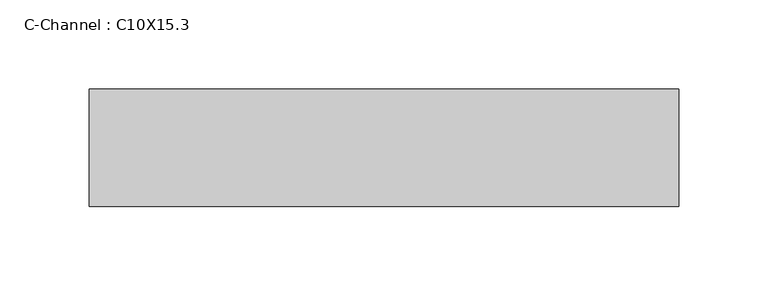
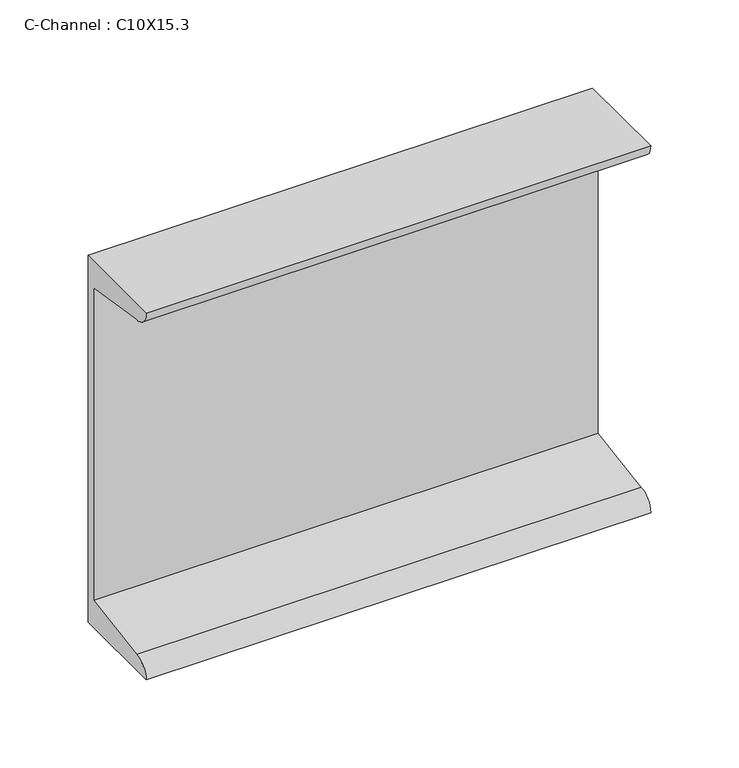
"""IFC4 building model written with IfcOpenShell, lengths in millimetres: beam geometry, C-Channel : C10X15.3."""

import ifcopenshell
import ifcopenshell.guid

model = None  # the IFC model being written
_history = None  # IfcOwnerHistory: only IFC2X3 demands one
_inside = {}  # id of a spatial element -> (the spatial element, [elements in it])
_under = {}  # id of a project, library or spatial element -> (it, [spatial elements below it])
_declared = {}  # id of a project -> (the project, [libraries it declares])
_typed = {}  # id of a type object -> (the type object, [elements of that type])
_made_of = {}  # id of a material, layer set ... -> (it, [elements and type objects made of it])


def new_model(schema):
    """Start an empty IFC model of exactly this schema.

    Asked for "IFC4X3", IfcOpenShell would pick the latest addendum, in which some entities
    have other attributes; the version numbers below select the first issue.
    IFC2X3 requires an IfcOwnerHistory on every rooted entity: one is made here for all.
    """
    global model, _history
    if schema == "IFC4X3":
        model = ifcopenshell.file(schema_version=(4, 3, 0, 0))
    else:
        model = ifcopenshell.file(schema=schema)
    _inside.clear()
    _under.clear()
    _declared.clear()
    _typed.clear()
    _made_of.clear()
    _history = None
    if model.schema == "IFC2X3":
        org = make("IfcOrganization", Name="unknown")
        user = make(
            "IfcPersonAndOrganization",
            ThePerson=make("IfcPerson", FamilyName="unknown"),
            TheOrganization=org,
        )
        app = make(
            "IfcApplication",
            ApplicationDeveloper=org,
            Version="unknown",
            ApplicationFullName="unknown",
            ApplicationIdentifier="unknown",
        )
        _history = make(
            "IfcOwnerHistory",
            OwningUser=user,
            OwningApplication=app,
            ChangeAction="ADDED",
            CreationDate=0,
        )
    return model


def make(cls, **values):
    """One entity of the class cls with the attributes given. An attribute that is None is left unset."""
    return model.create_entity(
        cls, **{name: value for name, value in values.items() if value is not None}
    )


def rooted(cls, **values):
    """An entity with a GlobalId (a new one), such as an element, a storey or a relation."""
    return make(cls, GlobalId=ifcopenshell.guid.new(), OwnerHistory=_history, **values)


def si_unit(unit_type, name, prefix=None):
    """IfcSIUnit, for example si_unit("LENGTHUNIT", "METRE", prefix="MILLI")."""
    return make("IfcSIUnit", UnitType=unit_type, Prefix=prefix, Name=name)


def assignment(units):
    """IfcUnitAssignment: the units of a project."""
    return None if units is None else make("IfcUnitAssignment", Units=units)


def point(xyz):
    """IfcCartesianPoint."""
    return None if xyz is None else make("IfcCartesianPoint", Coordinates=xyz)


def direction(xyz):
    """IfcDirection."""
    return None if xyz is None else make("IfcDirection", DirectionRatios=xyz)


def frame(location, z_axis=None, x_axis=None):
    """IfcAxis2Placement3D, a coordinate frame: its origin and axes. An axis left out is left unset."""
    return make(
        "IfcAxis2Placement3D",
        Location=point(location),
        Axis=direction(z_axis),
        RefDirection=direction(x_axis),
    )


def frame_2d(location, x_axis=None):
    """IfcAxis2Placement2D, a coordinate frame in the plane: its origin and x axis."""
    return make(
        "IfcAxis2Placement2D", Location=point(location), RefDirection=direction(x_axis)
    )


def origin():
    """The frame at (0, 0, 0) with its axes left unset."""
    return frame((0.0, 0.0, 0.0))


def place(relative_to, where):
    """IfcLocalPlacement: puts the frame where relative to a parent placement (None: the world)."""
    return make(
        "IfcLocalPlacement", PlacementRelTo=relative_to, RelativePlacement=where
    )


def context(
    kind, dimensions, precision=None, world=None, true_north=None, identifier=None
):
    """IfcGeometricRepresentationContext, for example the 3D "Model" context."""
    return make(
        "IfcGeometricRepresentationContext",
        ContextIdentifier=identifier,
        ContextType=kind,
        CoordinateSpaceDimension=dimensions,
        Precision=precision,
        WorldCoordinateSystem=world,
        TrueNorth=true_north,
    )


def project(units=None, contexts=None):
    """IfcProject with its units and contexts."""
    return rooted(
        "IfcProject",
        Name="project",
        RepresentationContexts=contexts,
        UnitsInContext=assignment(units),
    )


def spatial(cls, under=None, at=None, **own):
    """A site, building, storey or space (cls), placed at a placement, below another one or the project."""
    s = rooted(cls, ObjectPlacement=at, **own)
    if under is not None:
        _under.setdefault(under.id(), (under, []))[1].append(s)
    return s


def polyline(points):
    """IfcPolyline through the points."""
    return make("IfcPolyline", Points=[point(p) for p in points])


def circle_curve(where, radius):
    """IfcCircle in the frame where."""
    return make("IfcCircle", Position=where, Radius=radius)


def trimmed(basis, trim1, trim2, sense, master):
    """IfcTrimmedCurve: the piece of a basis curve between two trims."""
    return make(
        "IfcTrimmedCurve",
        BasisCurve=basis,
        Trim1=trim1,
        Trim2=trim2,
        SenseAgreement=sense,
        MasterRepresentation=master,
    )


def segment(curve, same_sense, transition):
    """IfcCompositeCurveSegment."""
    return make(
        "IfcCompositeCurveSegment",
        Transition=transition,
        SameSense=same_sense,
        ParentCurve=curve,
    )


def composite_curve(segments, self_intersect=None):
    """IfcCompositeCurve: segments joined end to end."""
    return make("IfcCompositeCurve", Segments=segments, SelfIntersect=self_intersect)


def outline(outer, holes=None, kind="AREA"):
    """IfcArbitraryClosedProfileDef: a profile drawn as a closed curve; with holes, ...WithVoids."""
    if holes is None:
        return make("IfcArbitraryClosedProfileDef", ProfileType=kind, OuterCurve=outer)
    return make(
        "IfcArbitraryProfileDefWithVoids",
        ProfileType=kind,
        OuterCurve=outer,
        InnerCurves=holes,
    )


def extrude(swept, where, along, depth):
    """IfcExtrudedAreaSolid: the profile swept, set in the frame where, extruded along a direction by depth."""
    return make(
        "IfcExtrudedAreaSolid",
        SweptArea=swept,
        Position=where,
        ExtrudedDirection=direction(along),
        Depth=depth,
    )


def shape(context_of_items, identifier, shape_type, items):
    """IfcShapeRepresentation: the items that make up one representation, for example the "Body"."""
    return make(
        "IfcShapeRepresentation",
        ContextOfItems=context_of_items,
        RepresentationIdentifier=identifier,
        RepresentationType=shape_type,
        Items=items,
    )


def source(mapping_origin, context_of_items, identifier, shape_type, items):
    """IfcRepresentationMap: a shape defined once, which mapped items show again and again."""
    return make(
        "IfcRepresentationMap",
        MappingOrigin=mapping_origin,
        MappedRepresentation=shape(context_of_items, identifier, shape_type, items),
    )


def transform(
    local_origin,
    x_axis=None,
    y_axis=None,
    z_axis=None,
    scale=None,
    scale2=None,
    scale3=None,
    uniform=True,
):
    """IfcCartesianTransformationOperator3D, or its non-uniform kind. x_axis, y_axis, z_axis: its Axis1, 2, 3."""
    if uniform:
        return make(
            "IfcCartesianTransformationOperator3D",
            Axis1=direction(x_axis),
            Axis2=direction(y_axis),
            LocalOrigin=point(local_origin),
            Scale=scale,
            Axis3=direction(z_axis),
        )
    return make(
        "IfcCartesianTransformationOperator3DnonUniform",
        Axis1=direction(x_axis),
        Axis2=direction(y_axis),
        LocalOrigin=point(local_origin),
        Scale=scale,
        Axis3=direction(z_axis),
        Scale2=scale2,
        Scale3=scale3,
    )


def mapped(mapping_source, mapping_target):
    """IfcMappedItem: shows the shape of a source again, moved by a transform."""
    return make(
        "IfcMappedItem", MappingSource=mapping_source, MappingTarget=mapping_target
    )


def made_of(thing, what):
    """Note that an element or type object is made of a material, layer set ...; save() writes the relation."""
    if what is not None:
        _made_of.setdefault(what.id(), (what, []))[1].append(thing)
    return thing


def element(
    cls,
    number,
    at=None,
    inside=None,
    cuts=None,
    type_object=None,
    material=None,
    context=None,
    identifier="Body",
    shape_type=None,
    held_by="IfcProductDefinitionShape",
    body=None,
    shapes=None,
    **own,
):
    """One element of the class cls, such as IfcWall. Its Tag is "e" and its number.

    at: its placement. inside: the storey or other place that contains it. cuts: it is an
    opening in that element (IfcRelVoidsElement). A single representation is given by context,
    identifier, shape_type and body (its items); several are given by shapes. held_by: the class
    of the entity that holds the representations. save() writes the other relations.
    """
    e = rooted(cls, Tag="e%d" % number, ObjectPlacement=at, **own)
    if body is not None:
        shapes = [shape(context, identifier, shape_type, body)]
    if shapes is not None:
        e.Representation = make(held_by, Representations=shapes)
    if inside is not None:
        _inside.setdefault(inside.id(), (inside, []))[1].append(e)
    if cuts is not None:
        rooted(
            "IfcRelVoidsElement", RelatingBuildingElement=cuts, RelatedOpeningElement=e
        )
    if type_object is not None:
        _typed.setdefault(type_object.id(), (type_object, []))[1].append(e)
    return made_of(e, material)


def aggregate(whole, parts):
    """IfcRelAggregates: a whole, such as a stair, and the parts it consists of."""
    return rooted("IfcRelAggregates", RelatingObject=whole, RelatedObjects=parts)


def save(model, path):
    """Write the relations noted so far, then the file.

    IfcRelAggregates (storeys below a building ...), IfcRelContainedInSpatialStructure (elements
    in a storey), IfcRelDefinesByType, IfcRelAssociatesMaterial and IfcRelDeclares: one each for
    every whole, place, type object, material and project.
    """
    for whole, parts in _under.values():
        aggregate(whole, parts)
    for where, things in _inside.values():
        rooted(
            "IfcRelContainedInSpatialStructure",
            RelatedElements=things,
            RelatingStructure=where,
        )
    for kind, things in _typed.values():
        rooted("IfcRelDefinesByType", RelatedObjects=things, RelatingType=kind)
    for what, things in _made_of.values():
        rooted("IfcRelAssociatesMaterial", RelatedObjects=things, RelatingMaterial=what)
    for by, libraries in _declared.values():
        rooted("IfcRelDeclares", RelatingContext=by, RelatedDefinitions=libraries)
    model.write(path)


def c_channel_c10x15_3_927e855d(model_context):
    return source(origin(), model_context, "Body", "SweptSolid", [
        extrude(outline(composite_curve([segment(polyline([(16.1036, 127.0), (16.1036, -127.0), (-49.9364, -127.0)]), True, "CONTINUOUS"), segment(trimmed(circle_curve(frame_2d((-38.862, -127.0)), 11.0744), [point((-49.9364, -127.0))], [point((-38.862, -115.9256))], False, "CARTESIAN"), True, "CONTINUOUS"), segment(polyline([(-38.862, -115.9256), (10.0076, -108.1854158), (10.0076, 108.1854158), (-38.862, 115.9256)]), True, "CONTINUOUS"), segment(trimmed(circle_curve(frame_2d((-38.862, 127.0)), 11.0744), [point((-38.862, 115.9256))], [point((-49.9364, 127.0))], False, "CARTESIAN"), True, "CONTINUOUS"), segment(polyline([(-49.9364, 127.0), (16.1036, 127.0)]), True, "CONTINUOUS")], self_intersect=False)), frame((-178.308, 0.0, 0.0), z_axis=(1.0, 0.0, 0.0), x_axis=(0.0, 1.0, 0.0)), (0.0, 0.0, 1.0), 330.708),
    ])


if __name__ == "__main__":
    model = new_model("IFC4")
    model_context = context("Model", 3, world=origin())
    ifc_project = project(units=[si_unit("LENGTHUNIT", "METRE", prefix="MILLI")], contexts=[model_context])
    site = spatial("IfcSite", under=ifc_project)
    building = spatial("IfcBuilding", under=site)
    placement = place(None, origin())
    c_channel_c10x15_3_shape = c_channel_c10x15_3_927e855d(model_context)
    element("IfcBeam", 1, ObjectType="C-Channel : C10X15.3", at=placement, inside=building, context=model_context, shape_type="MappedRepresentation", body=[
        mapped(c_channel_c10x15_3_shape, transform((0.0, 0.0, 0.0), x_axis=(1.0, 0.0, 0.0), y_axis=(0.0, 1.0, 0.0), z_axis=(0.0, 0.0, 1.0))),
    ])
    save(model, "model.ifc")

# Revit data of these elements
# Type "C-Channel : C10X15.3"
#   Assembly Code = "B10"
#   W = 15.3
#   Length [instance default] = 5' - 0"
#   bf = 0' - 2.6"
#   d = 0' - 10"
#   tf = 0' - 0.436"
#   tw = 0' - 0.24"
#   x = 0' - 0.634"
#   A = 0.0311111 SF
#   Structural Material [instance default] = Steel ASTM A36
# Element 1 (IfcBeam, "C-Channel : C10X15.3")
#   Structural Material = Steel ASTM A992
#   Materials on its faces: "Steel ASTM A992"
# Materials
#   "Steel ASTM A36": class "Metal", colour RGB 199 199 199, transparency 0, Description = "Structural steel, ASTM A36 Grade B, mill finish", Cost = 0
#   "Steel ASTM A992": class "Metal", colour RGB 199 199 199, transparency 0, Description = "Structural steel 50ksi", Cost = 0
